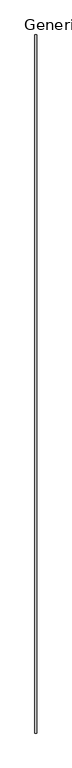
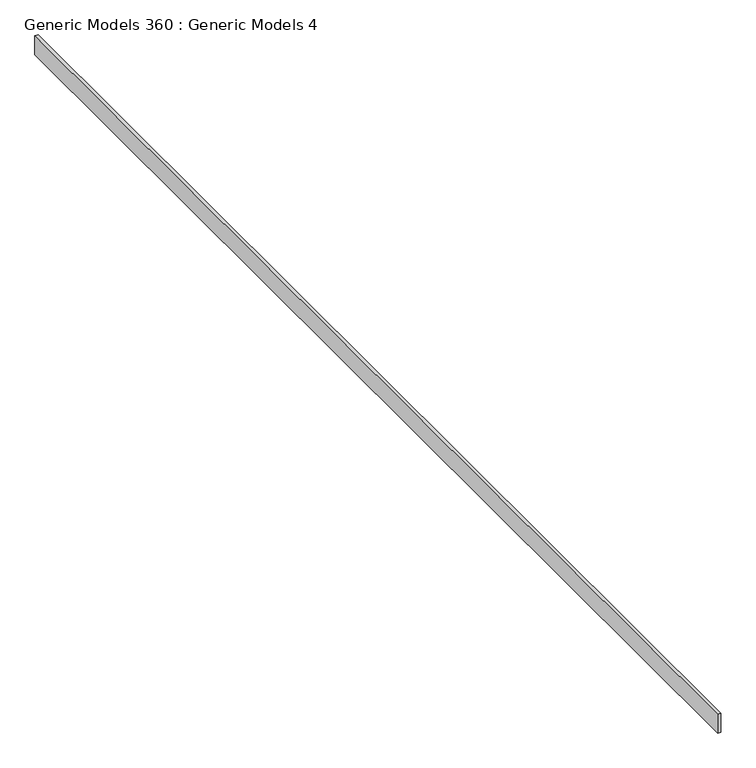
"""IFC4 building model written with IfcOpenShell, lengths in millimetres: proxy geometry, Generic Models 360 : Generic Models 4."""

from ifc_helpers import new_model, si_unit, frame, origin, place, context, project, spatial, polyline, outline, extrude, source, transform, mapped, element, save


def generic_models_360_generic_models_4_97fc5a00(model_context):
    return source(origin(), model_context, "Body", "SweptSolid", [
        extrude(outline(polyline([(-6338.8039395, -6864.9230338), (-6356.5236296, -6864.9230338), (-6356.5236296, -464.1230338), (-6338.8039395, -464.1230338), (-6338.8039395, -6864.9230338)])), frame((0.0, 0.0, 127253.8087534), z_axis=(0.0, 0.0, 1.0), x_axis=(1.0, 0.0, 0.0)), (0.0, 0.0, 1.0), 107.8244931),
    ])


if __name__ == "__main__":
    model = new_model("IFC4")
    model_context = context("Model", 3, world=origin())
    ifc_project = project(units=[si_unit("LENGTHUNIT", "METRE", prefix="MILLI")], contexts=[model_context])
    site = spatial("IfcSite", under=ifc_project)
    building = spatial("IfcBuilding", under=site)
    placement = place(None, origin())
    generic_models_360_generic_models_4_shape = generic_models_360_generic_models_4_97fc5a00(model_context)
    element("IfcBuildingElementProxy", 1, Name="Generic Models 360 : Generic Models 4", ObjectType="Generic Models 360 : Generic Models 4", at=placement, inside=building, context=model_context, shape_type="MappedRepresentation", body=[
        mapped(generic_models_360_generic_models_4_shape, transform((0.0, 0.0, 0.0), x_axis=(1.0, 0.0, 0.0), y_axis=(0.0, 1.0, 0.0), z_axis=(0.0, 0.0, 1.0))),
    ])
    save(model, "model.ifc")

# Revit data of these elements
# Element 1 (IfcBuildingElementProxy, "Generic Models 360 : Generic Models 4")
#   Materials on its faces: "_SOLID HARDWOOD STOCK"
# Materials
#   "_SOLID HARDWOOD STOCK": class "Generic", colour RGB 177 130 114, transparency 0, Cost = 0
